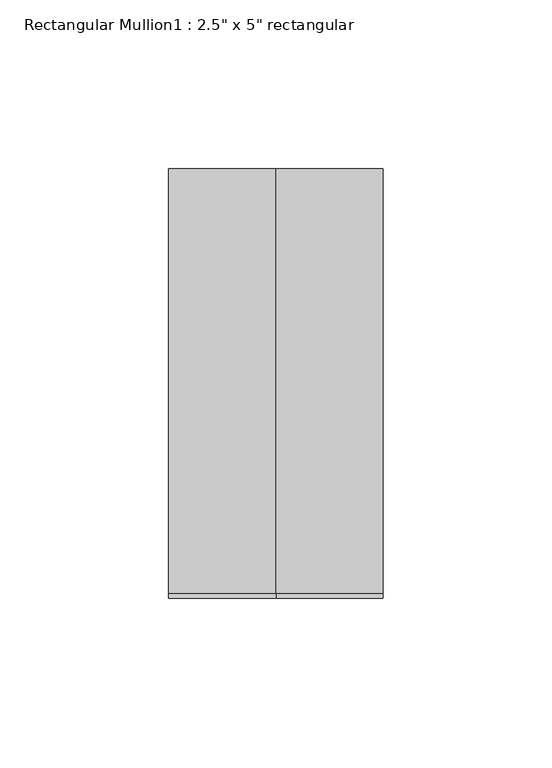
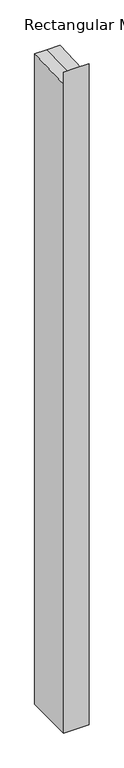
"""IFC4 building model written with IfcOpenShell, lengths in millimetres: member geometry."""

import ifcopenshell
import ifcopenshell.guid

model = None  # the IFC model being written
_history = None  # IfcOwnerHistory: only IFC2X3 demands one
_inside = {}  # id of a spatial element -> (the spatial element, [elements in it])
_under = {}  # id of a project, library or spatial element -> (it, [spatial elements below it])
_declared = {}  # id of a project -> (the project, [libraries it declares])
_typed = {}  # id of a type object -> (the type object, [elements of that type])
_made_of = {}  # id of a material, layer set ... -> (it, [elements and type objects made of it])


def new_model(schema):
    """Start an empty IFC model of exactly this schema.

    Asked for "IFC4X3", IfcOpenShell would pick the latest addendum, in which some entities
    have other attributes; the version numbers below select the first issue.
    IFC2X3 requires an IfcOwnerHistory on every rooted entity: one is made here for all.
    """
    global model, _history
    if schema == "IFC4X3":
        model = ifcopenshell.file(schema_version=(4, 3, 0, 0))
    else:
        model = ifcopenshell.file(schema=schema)
    _inside.clear()
    _under.clear()
    _declared.clear()
    _typed.clear()
    _made_of.clear()
    _history = None
    if model.schema == "IFC2X3":
        org = make("IfcOrganization", Name="unknown")
        user = make(
            "IfcPersonAndOrganization",
            ThePerson=make("IfcPerson", FamilyName="unknown"),
            TheOrganization=org,
        )
        app = make(
            "IfcApplication",
            ApplicationDeveloper=org,
            Version="unknown",
            ApplicationFullName="unknown",
            ApplicationIdentifier="unknown",
        )
        _history = make(
            "IfcOwnerHistory",
            OwningUser=user,
            OwningApplication=app,
            ChangeAction="ADDED",
            CreationDate=0,
        )
    return model


def make(cls, **values):
    """One entity of the class cls with the attributes given. An attribute that is None is left unset."""
    return model.create_entity(
        cls, **{name: value for name, value in values.items() if value is not None}
    )


def rooted(cls, **values):
    """An entity with a GlobalId (a new one), such as an element, a storey or a relation."""
    return make(cls, GlobalId=ifcopenshell.guid.new(), OwnerHistory=_history, **values)


def si_unit(unit_type, name, prefix=None):
    """IfcSIUnit, for example si_unit("LENGTHUNIT", "METRE", prefix="MILLI")."""
    return make("IfcSIUnit", UnitType=unit_type, Prefix=prefix, Name=name)


def assignment(units):
    """IfcUnitAssignment: the units of a project."""
    return None if units is None else make("IfcUnitAssignment", Units=units)


def point(xyz):
    """IfcCartesianPoint."""
    return None if xyz is None else make("IfcCartesianPoint", Coordinates=xyz)


def direction(xyz):
    """IfcDirection."""
    return None if xyz is None else make("IfcDirection", DirectionRatios=xyz)


def frame(location, z_axis=None, x_axis=None):
    """IfcAxis2Placement3D, a coordinate frame: its origin and axes. An axis left out is left unset."""
    return make(
        "IfcAxis2Placement3D",
        Location=point(location),
        Axis=direction(z_axis),
        RefDirection=direction(x_axis),
    )


def origin():
    """The frame at (0, 0, 0) with its axes left unset."""
    return frame((0.0, 0.0, 0.0))


def place(relative_to, where):
    """IfcLocalPlacement: puts the frame where relative to a parent placement (None: the world)."""
    return make(
        "IfcLocalPlacement", PlacementRelTo=relative_to, RelativePlacement=where
    )


def context(
    kind, dimensions, precision=None, world=None, true_north=None, identifier=None
):
    """IfcGeometricRepresentationContext, for example the 3D "Model" context."""
    return make(
        "IfcGeometricRepresentationContext",
        ContextIdentifier=identifier,
        ContextType=kind,
        CoordinateSpaceDimension=dimensions,
        Precision=precision,
        WorldCoordinateSystem=world,
        TrueNorth=true_north,
    )


def project(units=None, contexts=None):
    """IfcProject with its units and contexts."""
    return rooted(
        "IfcProject",
        Name="project",
        RepresentationContexts=contexts,
        UnitsInContext=assignment(units),
    )


def spatial(cls, under=None, at=None, **own):
    """A site, building, storey or space (cls), placed at a placement, below another one or the project."""
    s = rooted(cls, ObjectPlacement=at, **own)
    if under is not None:
        _under.setdefault(under.id(), (under, []))[1].append(s)
    return s


def faces_of(points, faces, orient=None, outer=None):
    """IfcFace entities. A face is a list of loops; a loop is a list of indices into points, from 0.

    orient and outer hold one flag for each loop. By default every Orientation is true, the
    first loop of a face is its IfcFaceOuterBound and the others are IfcFaceBound.
    """
    made = []
    for i, loops in enumerate(faces):
        bounds = []
        for j, loop in enumerate(loops):
            is_outer = j == 0 if outer is None else outer[i][j]
            bounds.append(
                make(
                    "IfcFaceOuterBound" if is_outer else "IfcFaceBound",
                    Bound=make("IfcPolyLoop", Polygon=[points[k] for k in loop]),
                    Orientation=True if orient is None else orient[i][j],
                )
            )
        made.append(make("IfcFace", Bounds=bounds))
    return made


def faceted_brep(points, faces, orient=None, outer=None, voids=None):
    """IfcFacetedBrep: a solid bounded by flat faces; with voids (closed shells), ...WithVoids."""
    shared = [point(p) for p in points]
    hull = make("IfcClosedShell", CfsFaces=faces_of(shared, faces, orient, outer))
    if voids is None:
        return make("IfcFacetedBrep", Outer=hull)
    return make(
        "IfcFacetedBrepWithVoids",
        Outer=hull,
        Voids=[
            make(cls, CfsFaces=faces_of(shared, fs, o, b)) for cls, fs, o, b in voids
        ],
    )


def shape(context_of_items, identifier, shape_type, items):
    """IfcShapeRepresentation: the items that make up one representation, for example the "Body"."""
    return make(
        "IfcShapeRepresentation",
        ContextOfItems=context_of_items,
        RepresentationIdentifier=identifier,
        RepresentationType=shape_type,
        Items=items,
    )


def source(mapping_origin, context_of_items, identifier, shape_type, items):
    """IfcRepresentationMap: a shape defined once, which mapped items show again and again."""
    return make(
        "IfcRepresentationMap",
        MappingOrigin=mapping_origin,
        MappedRepresentation=shape(context_of_items, identifier, shape_type, items),
    )


def transform(
    local_origin,
    x_axis=None,
    y_axis=None,
    z_axis=None,
    scale=None,
    scale2=None,
    scale3=None,
    uniform=True,
):
    """IfcCartesianTransformationOperator3D, or its non-uniform kind. x_axis, y_axis, z_axis: its Axis1, 2, 3."""
    if uniform:
        return make(
            "IfcCartesianTransformationOperator3D",
            Axis1=direction(x_axis),
            Axis2=direction(y_axis),
            LocalOrigin=point(local_origin),
            Scale=scale,
            Axis3=direction(z_axis),
        )
    return make(
        "IfcCartesianTransformationOperator3DnonUniform",
        Axis1=direction(x_axis),
        Axis2=direction(y_axis),
        LocalOrigin=point(local_origin),
        Scale=scale,
        Axis3=direction(z_axis),
        Scale2=scale2,
        Scale3=scale3,
    )


def mapped(mapping_source, mapping_target):
    """IfcMappedItem: shows the shape of a source again, moved by a transform."""
    return make(
        "IfcMappedItem", MappingSource=mapping_source, MappingTarget=mapping_target
    )


def made_of(thing, what):
    """Note that an element or type object is made of a material, layer set ...; save() writes the relation."""
    if what is not None:
        _made_of.setdefault(what.id(), (what, []))[1].append(thing)
    return thing


def element(
    cls,
    number,
    at=None,
    inside=None,
    cuts=None,
    type_object=None,
    material=None,
    context=None,
    identifier="Body",
    shape_type=None,
    held_by="IfcProductDefinitionShape",
    body=None,
    shapes=None,
    **own,
):
    """One element of the class cls, such as IfcWall. Its Tag is "e" and its number.

    at: its placement. inside: the storey or other place that contains it. cuts: it is an
    opening in that element (IfcRelVoidsElement). A single representation is given by context,
    identifier, shape_type and body (its items); several are given by shapes. held_by: the class
    of the entity that holds the representations. save() writes the other relations.
    """
    e = rooted(cls, Tag="e%d" % number, ObjectPlacement=at, **own)
    if body is not None:
        shapes = [shape(context, identifier, shape_type, body)]
    if shapes is not None:
        e.Representation = make(held_by, Representations=shapes)
    if inside is not None:
        _inside.setdefault(inside.id(), (inside, []))[1].append(e)
    if cuts is not None:
        rooted(
            "IfcRelVoidsElement", RelatingBuildingElement=cuts, RelatedOpeningElement=e
        )
    if type_object is not None:
        _typed.setdefault(type_object.id(), (type_object, []))[1].append(e)
    return made_of(e, material)


def aggregate(whole, parts):
    """IfcRelAggregates: a whole, such as a stair, and the parts it consists of."""
    return rooted("IfcRelAggregates", RelatingObject=whole, RelatedObjects=parts)


def save(model, path):
    """Write the relations noted so far, then the file.

    IfcRelAggregates (storeys below a building ...), IfcRelContainedInSpatialStructure (elements
    in a storey), IfcRelDefinesByType, IfcRelAssociatesMaterial and IfcRelDeclares: one each for
    every whole, place, type object, material and project.
    """
    for whole, parts in _under.values():
        aggregate(whole, parts)
    for where, things in _inside.values():
        rooted(
            "IfcRelContainedInSpatialStructure",
            RelatedElements=things,
            RelatingStructure=where,
        )
    for kind, things in _typed.values():
        rooted("IfcRelDefinesByType", RelatedObjects=things, RelatingType=kind)
    for what, things in _made_of.values():
        rooted("IfcRelAssociatesMaterial", RelatedObjects=things, RelatingMaterial=what)
    for by, libraries in _declared.values():
        rooted("IfcRelDeclares", RelatingContext=by, RelatedDefinitions=libraries)
    model.write(path)


def member_780b0c29(model_context):
    return source(origin(), model_context, "Body", "Brep", [
        faceted_brep([(31.75, 63.5, -1733.5500228), (31.75, -63.5, -1733.5500228), (-31.75, -63.5, -1733.5500228), (-31.75, 63.5, -1733.5500228), (-31.75, 63.5, 2.5257955), (0.0, 63.5, 2.5257955), (31.75, 63.5, 2.5257955), (-31.75, -63.5, 30.4748075), (-31.75, -62.1741259, -2.5237591), (31.75, -63.5, 30.4748075), (0.0, -63.5, 30.4748075), (31.75, -62.1741259, -2.5237591), (0.0, -62.1741259, -2.5237591)], [[[0, 1, 2, 3]], [[4, 5, 6, 0, 3]], [[7, 8, 4, 3, 2]], [[9, 10, 7, 2, 1]], [[6, 11, 9, 1, 0]], [[6, 5, 12, 11]], [[5, 4, 8, 12]], [[8, 7, 10, 12]], [[10, 9, 11, 12]]]),
    ])


if __name__ == "__main__":
    model = new_model("IFC4")
    model_context = context("Model", 3, world=origin())
    ifc_project = project(units=[si_unit("LENGTHUNIT", "METRE", prefix="MILLI")], contexts=[model_context])
    site = spatial("IfcSite", under=ifc_project)
    building = spatial("IfcBuilding", under=site)
    placement = place(None, origin())
    member_shape = member_780b0c29(model_context)
    element("IfcMember", 1, ObjectType="Rectangular Mullion1 : 2.5\" x 5\" rectangular", at=placement, inside=building, context=model_context, shape_type="MappedRepresentation", body=[
        mapped(member_shape, transform((0.0, 0.0, 0.0), x_axis=(1.0, 0.0, 0.0), y_axis=(0.0, 1.0, 0.0), z_axis=(0.0, 0.0, 1.0))),
    ])
    save(model, "model.ifc")

# Revit data of these elements
# Type "Rectangular Mullion1 : 2.5\" x 5\" rectangular"
#   built-in parameter 1007304 = 0.416667 (stored number, unit not read)
#   built-in parameter 1007301 = 0.104167 (stored number, unit not read)
#   built-in parameter 1007300 = 0.104167 (stored number, unit not read)
# Element 1 (IfcMember, "Rectangular Mullion1 : 2.5\" x 5\" rectangular")
#   Materials on its faces: "support-frame"
# Materials
#   "support-frame": class "Unassigned", colour RGB 233 233 233, transparency 0, Cost = 0
